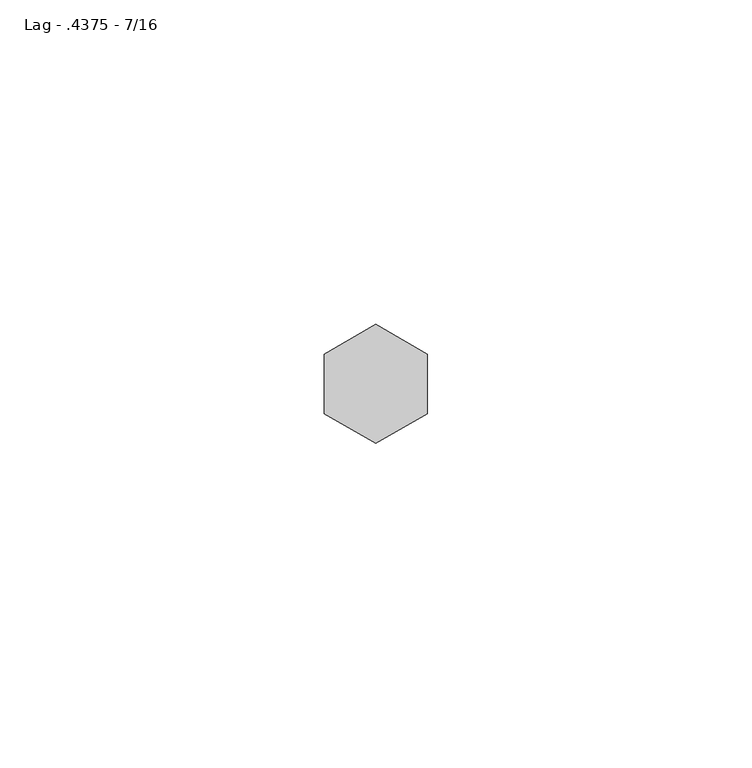
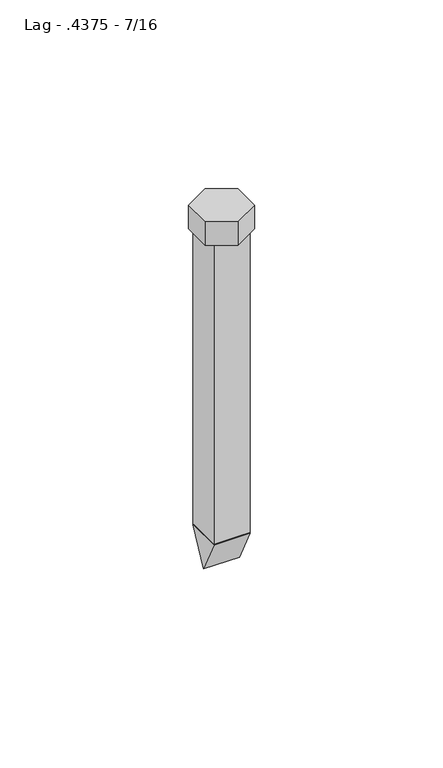
"""IFC4 building model written with IfcOpenShell, lengths in millimetres: fastener geometry, 060523 - W_P_C - Fastenings - Generic - SQUARE : Lag - .4375 - 7/16."""

from ifc_helpers import new_model, si_unit, frame, origin, origin_with_axes, place, context, project, spatial, polyline, outline, extrude, source, transform, mapped, element, save


def lag_4375_7_16_16092e99(model_context):
    return source(origin(), model_context, "Body", "SweptSolid", [
        extrude(outline(polyline([(0.0, -113.109375), (-5.7546875, -101.6), (5.7546875, -101.6), (0.0, -113.109375)])), frame((-5.7546875, 0.0, 0.0), z_axis=(1.0, 0.0, 0.0), x_axis=(0.0, 1.0, 0.0)), (0.0, 0.0, 1.0), 11.509375),
        extrude(outline(polyline([(-7.9375, 4.5827178), (0.0, 9.1654355), (7.9375, 4.5827178), (7.9375, -4.5827178), (0.0, -9.1654355), (-7.9375, -4.5827178), (-7.9375, 4.5827178)])), origin_with_axes(), (0.0, 0.0, 1.0), 8.0367187),
        extrude(outline(polyline([(-5.7546875, 5.7546875), (5.7546875, 5.7546875), (5.7546875, -5.7546875), (-5.7546875, -5.7546875), (-5.7546875, 5.7546875)])), frame((0.0, 0.0, -101.6), z_axis=(0.0, 0.0, 1.0), x_axis=(1.0, 0.0, 0.0)), (0.0, 0.0, 1.0), 101.6),
    ])


if __name__ == "__main__":
    model = new_model("IFC4")
    model_context = context("Model", 3, world=origin())
    ifc_project = project(units=[si_unit("LENGTHUNIT", "METRE", prefix="MILLI")], contexts=[model_context])
    site = spatial("IfcSite", under=ifc_project)
    building = spatial("IfcBuilding", under=site)
    placement = place(None, origin())
    lag_4375_7_16_shape = lag_4375_7_16_16092e99(model_context)
    element("IfcFastener", 1, ObjectType="060523 - W_P_C - Fastenings - Generic - SQUARE : Lag - .4375 - 7/16", at=placement, inside=building, context=model_context, shape_type="MappedRepresentation", body=[
        mapped(lag_4375_7_16_shape, transform((0.0, 0.0, 0.0), x_axis=(1.0, 0.0, 0.0), y_axis=(0.0, 1.0, 0.0), z_axis=(0.0, 0.0, 1.0))),
    ])
    save(model, "model.ifc")

# Revit data of these elements
# Type "060523 - W_P_C - Fastenings - Generic - SQUARE : Lag - .4375 - 7/16"
#   Washer_Thickness = 0' - 0 27/256"
#   Washer Radius = 0' - 0 139/256"
#   Washer Offset - Head = 0' - 0"
#   Washer Offset = 0' - 0"
#   Thickness_of_Substrate [instance default] = 0' - 1"
#   Side = 0' - 0.36133"
#   Radius = 0' - 0 29/128"
#   Length [instance default] = 0' - 4"
#   Head Size = 0' - 0 5/8"
#   Head Radius = 0' - 0 5/16"
#   Head Height = 0' - 0 81/256"
#   Double Diameter = 0' - 0 29/32"
#   Diameter = 0' - 0 29/64"
#   Default Elevation = 4' - 0"
#   Washer_Nut_Visibility = no
#   Washer_Head_Visibility = no
#   Round_Head_Visibility = no
#   Point Visibility = yes
#   Nut_Visibility = no
#   Hex_Head_Visiblilty = yes
#   Washer Material = none
#   Bolt Material (Size) = AT SILL - FASTENER AT 24" O.C.
# Element 1 (IfcFastener, "060523 - W_P_C - Fastenings - Generic - SQUARE : Lag - .4375 - 7/16")
#   Materials on its faces: "AT SILL - FASTENER AT 24\" O.C."
# Materials
#   "AT SILL - FASTENER AT 24\" O.C.": class "Generic", colour RGB 120 120 120, transparency 0, Cost = 0
